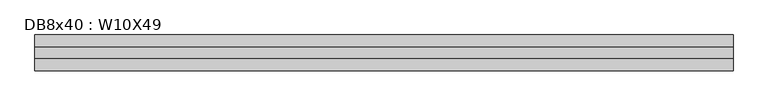
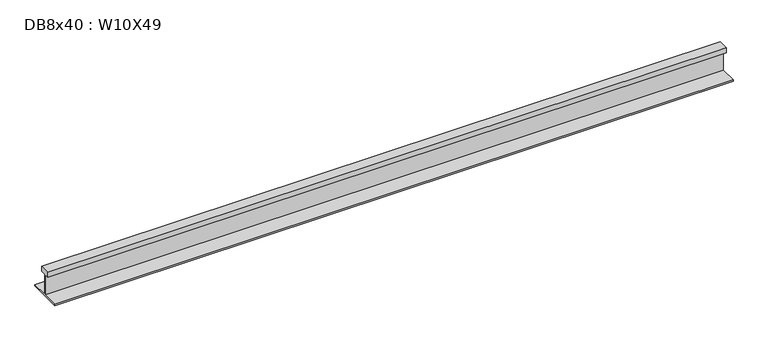
"""IFC4 building model written with IfcOpenShell, lengths in millimetres: beam geometry, DB8x40 : W10X49."""

from ifc_helpers import new_model, si_unit, frame, origin, place, context, project, spatial, polyline, outline, extrude, source, transform, mapped, element, save


def db8x40_w10x49_6679a255(model_context):
    return source(origin(), model_context, "Body", "SweptSolid", [
        extrude(outline(polyline([(38.1, 144.3355), (38.1, 106.2355), (2.921, 106.2355), (2.921, -49.53), (127.0, -49.53), (127.0, -59.182), (-127.0, -59.182), (-127.0, -49.53), (-2.921, -49.53), (-2.921, 106.2355), (-38.1, 106.2355), (-38.1, 144.3355), (38.1, 144.3355)])), frame((-2479.929, 0.0, 0.0), z_axis=(1.0, 0.0, 0.0), x_axis=(0.0, 1.0, 0.0)), (0.0, 0.0, 1.0), 4959.858),
    ])


if __name__ == "__main__":
    model = new_model("IFC4")
    model_context = context("Model", 3, world=origin())
    ifc_project = project(units=[si_unit("LENGTHUNIT", "METRE", prefix="MILLI")], contexts=[model_context])
    site = spatial("IfcSite", under=ifc_project)
    building = spatial("IfcBuilding", under=site)
    placement = place(None, origin())
    db8x40_w10x49_shape = db8x40_w10x49_6679a255(model_context)
    element("IfcBeam", 1, ObjectType="DB8x40 : W10X49", at=placement, inside=building, context=model_context, shape_type="MappedRepresentation", body=[
        mapped(db8x40_w10x49_shape, transform((0.0, 0.0, 0.0), x_axis=(1.0, 0.0, 0.0), y_axis=(0.0, 1.0, 0.0), z_axis=(0.0, 0.0, 1.0))),
    ])
    save(model, "model.ifc")

# Revit data of these elements
# Type "DB8x40 : W10X49"
#   Assembly Code = "B10"
#   W = 53
#   Length [instance default] = 5' - 0"
#   bf = 0' - 10"
#   d = 1' - 0.1"
#   k = 0' - 1 3/8"
#   k2 = 0' - 0.8"
#   tf = 0' - 0.575"
#   tw = 0' - 0.345"
#   A = 0.108333 SF
#   Structural Material [instance default] = Steel ASTM A992
# Element 1 (IfcBeam, "DB8x40 : W10X49")
#   Materials on its faces: "Steel ASTM A992"
# Materials
#   "Steel ASTM A992": class "Metal", colour RGB 199 199 199, transparency 0, Description = "Structural steel 50ksi", Cost = 0
